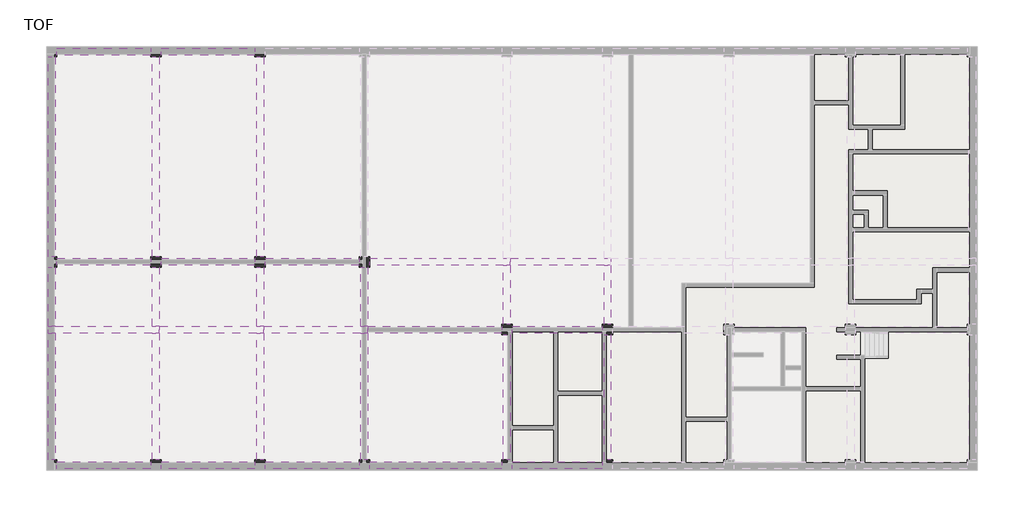
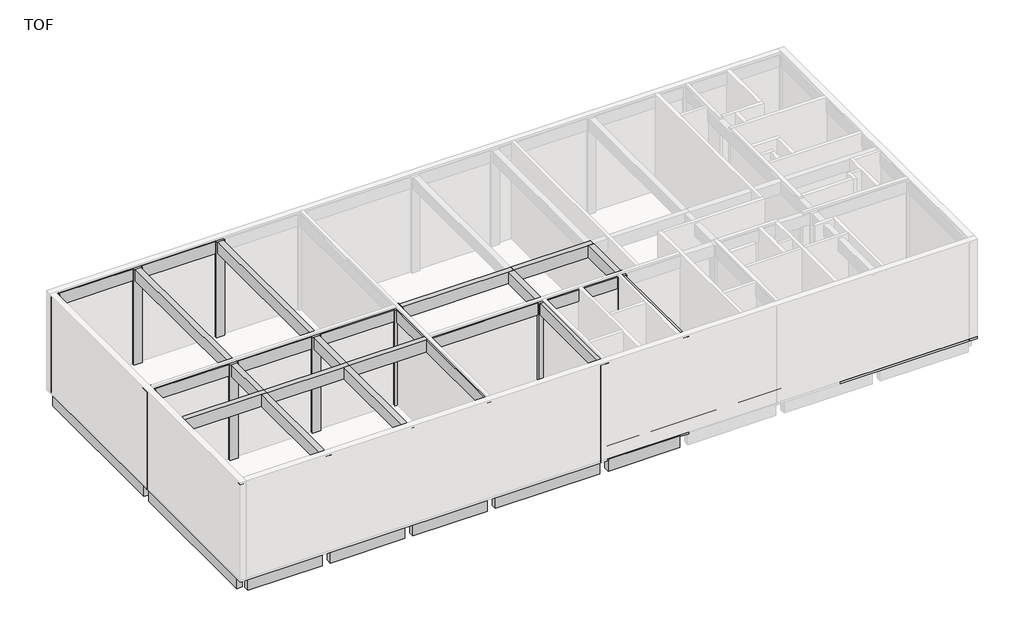
# One storey, part 2 of 3: 41 beams, 15 columns, 3 slabs.
"""IFC4 building model written with IfcOpenShell, lengths in millimetres."""

from ifc_helpers import new_model, si_unit, frame, origin, origin_with_axes, place, context, project, spatial, polyline, outline, extrude, faceted_brep, element, save

model = new_model("IFC4")

# Units and contexts
model_context = context("Model", 3, world=origin())
ifc_project = project(units=[si_unit("LENGTHUNIT", "METRE", prefix="MILLI")], contexts=[model_context])

# Site, building, storey
site = spatial("IfcSite", under=ifc_project)
building = spatial("IfcBuilding", under=site)
storey = spatial("IfcBuildingStorey", under=building, Name="TOF", Elevation=150.0)

# Beams
placement = place(None, origin())
element("IfcBeam", 1, ObjectType="RC Beam_Rectangular : H_SB_ACB_B400xH900", at=placement, inside=storey, context=model_context, shape_type="SweptSolid", body=[
    extrude(outline(polyline([(124.7, 12616.5208589), (-275.3, 12616.5208589), (-275.3, 24116.5208589), (124.7, 24116.5208589), (124.7, 12616.5208589)])), frame((0.0, 0.0, -900.0), z_axis=(0.0, 0.0, 1.0), x_axis=(1.0, 0.0, 0.0)), (0.0, 0.0, 1.0), 900.0),
])
element("IfcBeam", 2, ObjectType="RC Beam_Rectangular : H_SB_ACB_B400xH900", at=placement, inside=storey, context=model_context, shape_type="SweptSolid", body=[
    extrude(outline(polyline([(124.7, 916.5208589), (-275.3, 916.5208589), (-275.3, 12016.5208589), (124.7, 12016.5208589), (124.7, 916.5208589)])), frame((0.0, 0.0, -900.0), z_axis=(0.0, 0.0, 1.0), x_axis=(1.0, 0.0, 0.0)), (0.0, 0.0, 1.0), 900.0),
])
element("IfcBeam", 3, ObjectType="RC Beam_Rectangular : H_SB_ACB_B400xH900", at=placement, inside=storey, context=model_context, shape_type="SweptSolid", body=[
    extrude(outline(polyline([(5624.7, 24616.5208589), (5624.7, 24216.5208589), (224.7, 24216.5208589), (224.7, 24616.5208589), (5624.7, 24616.5208589)])), frame((0.0, 0.0, -900.0), z_axis=(0.0, 0.0, 1.0), x_axis=(1.0, 0.0, 0.0)), (0.0, 0.0, 1.0), 900.0),
])
element("IfcBeam", 4, ObjectType="RC Beam_Rectangular : H_SB_ACB_B400xH900", at=placement, inside=storey, context=model_context, shape_type="SweptSolid", body=[
    extrude(outline(polyline([(6224.7, 24216.5208589), (6224.7, 24616.5208589), (11624.7, 24616.5208589), (11624.7, 24216.5208589), (6224.7, 24216.5208589)])), frame((0.0, 0.0, -900.0), z_axis=(0.0, 0.0, 1.0), x_axis=(1.0, 0.0, 0.0)), (0.0, 0.0, 1.0), 900.0),
])
element("IfcBeam", 5, ObjectType="RC Beam_Rectangular : H_SB_ACB_B400xH900", at=placement, inside=storey, context=model_context, shape_type="SweptSolid", body=[
    extrude(outline(polyline([(224.7, 416.5208589), (224.7, 816.5208589), (5624.7, 816.5208589), (5624.7, 416.5208589), (224.7, 416.5208589)])), frame((0.0, 0.0, -900.0), z_axis=(0.0, 0.0, 1.0), x_axis=(1.0, 0.0, 0.0)), (0.0, 0.0, 1.0), 900.0),
])
element("IfcBeam", 6, ObjectType="RC Beam_Rectangular : H_SB_ACB_B400xH900", at=placement, inside=storey, context=model_context, shape_type="SweptSolid", body=[
    extrude(outline(polyline([(6224.7, 416.5208589), (6224.7, 816.5208589), (11624.7, 816.5208589), (11624.7, 416.5208589), (6224.7, 416.5208589)])), frame((0.0, 0.0, -900.0), z_axis=(0.0, 0.0, 1.0), x_axis=(1.0, 0.0, 0.0)), (0.0, 0.0, 1.0), 900.0),
])
element("IfcBeam", 7, ObjectType="RC Beam_Rectangular : H_SB_ACB_B400xH900", at=placement, inside=storey, context=model_context, shape_type="SweptSolid", body=[
    extrude(outline(polyline([(12224.7, 416.5208589), (12224.7, 816.5208589), (17624.7, 816.5208589), (17624.7, 416.5208589), (12224.7, 416.5208589)])), frame((0.0, 0.0, -900.0), z_axis=(0.0, 0.0, 1.0), x_axis=(1.0, 0.0, 0.0)), (0.0, 0.0, 1.0), 900.0),
])
element("IfcBeam", 8, ObjectType="RC Beam_Rectangular : H_SB_ACB_B400xH900", at=placement, inside=storey, context=model_context, shape_type="SweptSolid", body=[
    extrude(outline(polyline([(18224.7, 416.5208589), (18224.7, 816.5208589), (25824.7, 816.5208589), (25824.7, 416.5208589), (18224.7, 416.5208589)])), frame((0.0, 0.0, -900.0), z_axis=(0.0, 0.0, 1.0), x_axis=(1.0, 0.0, 0.0)), (0.0, 0.0, 1.0), 900.0),
])
element("IfcBeam", 9, ObjectType="RC Beam_Rectangular : H_SB_ACB_B400xH900", at=placement, inside=storey, context=model_context, shape_type="SweptSolid", body=[
    extrude(outline(polyline([(26424.7, 416.5208589), (26424.7, 816.5208589), (31624.7, 816.5208589), (31624.7, 416.5208589), (26424.7, 416.5208589)])), frame((0.0, 0.0, -900.0), z_axis=(0.0, 0.0, 1.0), x_axis=(1.0, 0.0, 0.0)), (0.0, 0.0, 1.0), 900.0),
])
element("IfcBeam", 10, ObjectType="RC Beam_Rectangular : H_SB_ACB_B400xH900", at=placement, inside=storey, context=model_context, shape_type="SweptSolid", body=[
    extrude(outline(polyline([(224.7, 12116.5208589), (224.7, 12516.5208589), (5624.7, 12516.5208589), (5624.7, 12116.5208589), (224.7, 12116.5208589)])), frame((0.0, 0.0, 6600.0), z_axis=(0.0, 0.0, 1.0), x_axis=(1.0, 0.0, 0.0)), (0.0, 0.0, 1.0), 900.0),
])
element("IfcBeam", 11, ObjectType="RC Beam_Rectangular : H_SB_ACB_B400xH900", at=placement, inside=storey, context=model_context, shape_type="SweptSolid", body=[
    extrude(outline(polyline([(6224.7, 12116.5208589), (6224.7, 12516.5208589), (11624.7, 12516.5208589), (11624.7, 12116.5208589), (6224.7, 12116.5208589)])), frame((0.0, 0.0, 6600.0), z_axis=(0.0, 0.0, 1.0), x_axis=(1.0, 0.0, 0.0)), (0.0, 0.0, 1.0), 900.0),
])
element("IfcBeam", 12, ObjectType="RC Beam_Rectangular : H_SB_ACB_B400xH900", at=placement, inside=storey, context=model_context, shape_type="SweptSolid", body=[
    extrude(outline(polyline([(12224.7, 12116.5208589), (12224.7, 12516.5208589), (17624.7, 12516.5208589), (17624.7, 12116.5208589), (12224.7, 12116.5208589)])), frame((0.0, 0.0, 6600.0), z_axis=(0.0, 0.0, 1.0), x_axis=(1.0, 0.0, 0.0)), (0.0, 0.0, 1.0), 900.0),
])
element("IfcBeam", 13, ObjectType="RC Beam_Rectangular : H_SB_ACB_B400xH900", at=placement, inside=storey, context=model_context, shape_type="Brep", body=[
    faceted_brep([(26324.7, 12116.5208589, 7500.0), (26324.7, 12516.5208589, 7500.0), (25924.7, 12516.5208589, 7500.0), (18224.7, 12516.5208589, 7500.0), (18224.7, 12116.5208589, 7500.0), (25924.7, 12116.5208589, 7500.0), (26324.7, 12116.5208589, 6600.0), (18224.7, 12116.5208589, 6600.0), (25924.7, 12116.5208589, 6600.0), (26324.7, 12516.5208589, 6600.0), (18224.7, 12516.5208589, 6600.0), (25924.7, 12516.5208589, 6600.0)], [[[0, 1, 2, 3, 4, 5]], [[6, 0, 5, 4, 7, 8]], [[9, 6, 8, 7, 10, 11]], [[1, 9, 11, 10, 3, 2]], [[4, 3, 10, 7]], [[1, 0, 6, 9]]]),
])
element("IfcBeam", 14, ObjectType="RC Beam_Rectangular : H_SB_ACB_B400xH900", at=placement, inside=storey, context=model_context, shape_type="Brep", body=[
    faceted_brep([(32124.7, 12116.5208589, 7500.0), (32124.7, 12516.5208589, 7500.0), (31724.7, 12516.5208589, 7500.0), (26324.7, 12516.5208589, 7500.0), (26324.7, 12116.5208589, 7500.0), (31724.7, 12116.5208589, 7500.0), (32124.7, 12116.5208589, 6600.0), (26324.7, 12116.5208589, 6600.0), (31724.7, 12116.5208589, 6600.0), (32124.7, 12516.5208589, 6600.0), (26324.7, 12516.5208589, 6600.0), (31724.7, 12516.5208589, 6600.0)], [[[0, 1, 2, 3, 4, 5]], [[6, 0, 5, 4, 7, 8]], [[9, 6, 8, 7, 10, 11]], [[1, 9, 11, 10, 3, 2]], [[1, 0, 6, 9]], [[4, 3, 10, 7]]]),
])
element("IfcBeam", 15, ObjectType="RC Beam_Rectangular : H_SB_ACB_B400xH900", at=placement, inside=storey, context=model_context, shape_type="SweptSolid", body=[
    extrude(outline(polyline([(224.7, 24216.5208589), (224.7, 24616.5208589), (5624.7, 24616.5208589), (5624.7, 24216.5208589), (224.7, 24216.5208589)])), frame((0.0, 0.0, 6600.0), z_axis=(0.0, 0.0, 1.0), x_axis=(1.0, 0.0, 0.0)), (0.0, 0.0, 1.0), 900.0),
])
element("IfcBeam", 16, ObjectType="RC Beam_Rectangular : H_SB_ACB_B400xH900", at=placement, inside=storey, context=model_context, shape_type="SweptSolid", body=[
    extrude(outline(polyline([(6224.7, 24216.5208589), (6224.7, 24616.5208589), (11624.7, 24616.5208589), (11624.7, 24216.5208589), (6224.7, 24216.5208589)])), frame((0.0, 0.0, 6600.0), z_axis=(0.0, 0.0, 1.0), x_axis=(1.0, 0.0, 0.0)), (0.0, 0.0, 1.0), 900.0),
])
element("IfcBeam", 17, ObjectType="RC Beam_Rectangular : H_SB_ACB_B400xH900", at=placement, inside=storey, context=model_context, shape_type="Brep", body=[
    faceted_brep([(-275.3, 8616.5208589, 7500.0), (-275.3, 8216.5208589, 7500.0), (124.7, 8216.5208589, 7500.0), (5724.7, 8216.5208589, 7500.0), (6124.7, 8216.5208589, 7500.0), (6124.7, 8616.5208589, 7500.0), (5724.7, 8616.5208589, 7500.0), (124.7, 8616.5208589, 7500.0), (-275.3, 8216.5208589, 6600.0), (124.7, 8216.5208589, 6600.0), (5724.7, 8216.5208589, 6600.0), (6124.7, 8216.5208589, 6600.0), (-275.3, 8616.5208589, 6600.0), (124.7, 8616.5208589, 6600.0), (5724.7, 8616.5208589, 6600.0), (6124.7, 8616.5208589, 6600.0)], [[[0, 1, 2, 3, 4, 5, 6, 7]], [[1, 8, 9, 10, 11, 4, 3, 2]], [[8, 12, 13, 14, 15, 11, 10, 9]], [[12, 0, 7, 6, 5, 15, 14, 13]], [[1, 0, 12, 8]], [[5, 4, 11, 15]]]),
])
element("IfcBeam", 18, ObjectType="RC Beam_Rectangular : H_SB_ACB_B400xH900", at=placement, inside=storey, context=model_context, shape_type="Brep", body=[
    faceted_brep([(12124.7, 8216.5208589, 7500.0), (12124.7, 8616.5208589, 7500.0), (11724.7, 8616.5208589, 7500.0), (6124.7, 8616.5208589, 7500.0), (6124.7, 8216.5208589, 7500.0), (11724.7, 8216.5208589, 7500.0), (12124.7, 8216.5208589, 6600.0), (6124.7, 8216.5208589, 6600.0), (11724.7, 8216.5208589, 6600.0), (12124.7, 8616.5208589, 6600.0), (6124.7, 8616.5208589, 6600.0), (11724.7, 8616.5208589, 6600.0)], [[[0, 1, 2, 3, 4, 5]], [[6, 0, 5, 4, 7, 8]], [[9, 6, 8, 7, 10, 11]], [[1, 9, 11, 10, 3, 2]], [[1, 0, 6, 9]], [[4, 3, 10, 7]]]),
])
element("IfcBeam", 19, ObjectType="RC Beam_Rectangular : H_SB_ACB_B400xH900", at=placement, inside=storey, context=model_context, shape_type="Brep", body=[
    faceted_brep([(18124.7, 8216.5208589, 7500.0), (18124.7, 8616.5208589, 7500.0), (17724.7, 8616.5208589, 7500.0), (12124.7, 8616.5208589, 7500.0), (12124.7, 8216.5208589, 7500.0), (17724.7, 8216.5208589, 7500.0), (18124.7, 8216.5208589, 6600.0), (12124.7, 8216.5208589, 6600.0), (17724.7, 8216.5208589, 6600.0), (18124.7, 8616.5208589, 6600.0), (12124.7, 8616.5208589, 6600.0), (17724.7, 8616.5208589, 6600.0)], [[[0, 1, 2, 3, 4, 5]], [[6, 0, 5, 4, 7, 8]], [[9, 6, 8, 7, 10, 11]], [[1, 9, 11, 10, 3, 2]], [[1, 0, 6, 9]], [[4, 3, 10, 7]]]),
])
element("IfcBeam", 20, ObjectType="RC Beam_Rectangular : H_SB_ACB_B400xH900", at=placement, inside=storey, context=model_context, shape_type="SweptSolid", body=[
    extrude(outline(polyline([(18124.7, 8216.5208589), (18124.7, 8616.5208589), (25824.7, 8616.5208589), (25824.7, 8216.5208589), (18124.7, 8216.5208589)])), frame((0.0, 0.0, 6600.0), z_axis=(0.0, 0.0, 1.0), x_axis=(1.0, 0.0, 0.0)), (0.0, 0.0, 1.0), 900.0),
])
element("IfcBeam", 21, ObjectType="RC Beam_Rectangular : H_SB_ACB_B400xH900", at=placement, inside=storey, context=model_context, shape_type="SweptSolid", body=[
    extrude(outline(polyline([(26424.7, 8216.5208589), (26424.7, 8616.5208589), (31624.7, 8616.5208589), (31624.7, 8216.5208589), (26424.7, 8216.5208589)])), frame((0.0, 0.0, 6600.0), z_axis=(0.0, 0.0, 1.0), x_axis=(1.0, 0.0, 0.0)), (0.0, 0.0, 1.0), 900.0),
])
element("IfcBeam", 22, ObjectType="RC Beam_Rectangular : H_SB_ACB_B400xH900", at=placement, inside=storey, context=model_context, shape_type="SweptSolid", body=[
    extrude(outline(polyline([(224.7, 416.5208589), (224.7, 816.5208589), (5624.7, 816.5208589), (5624.7, 416.5208589), (224.7, 416.5208589)])), frame((0.0, 0.0, 6600.0), z_axis=(0.0, 0.0, 1.0), x_axis=(1.0, 0.0, 0.0)), (0.0, 0.0, 1.0), 900.0),
])
element("IfcBeam", 23, ObjectType="RC Beam_Rectangular : H_SB_ACB_B400xH900", at=placement, inside=storey, context=model_context, shape_type="SweptSolid", body=[
    extrude(outline(polyline([(6224.7, 416.5208589), (6224.7, 816.5208589), (11624.7, 816.5208589), (11624.7, 416.5208589), (6224.7, 416.5208589)])), frame((0.0, 0.0, 6600.0), z_axis=(0.0, 0.0, 1.0), x_axis=(1.0, 0.0, 0.0)), (0.0, 0.0, 1.0), 900.0),
])
element("IfcBeam", 24, ObjectType="RC Beam_Rectangular : H_SB_ACB_B400xH900", at=placement, inside=storey, context=model_context, shape_type="SweptSolid", body=[
    extrude(outline(polyline([(12224.7, 416.5208589), (12224.7, 816.5208589), (17624.7, 816.5208589), (17624.7, 416.5208589), (12224.7, 416.5208589)])), frame((0.0, 0.0, 6600.0), z_axis=(0.0, 0.0, 1.0), x_axis=(1.0, 0.0, 0.0)), (0.0, 0.0, 1.0), 900.0),
])
element("IfcBeam", 25, ObjectType="RC Beam_Rectangular : H_SB_ACB_B400xH900", at=placement, inside=storey, context=model_context, shape_type="SweptSolid", body=[
    extrude(outline(polyline([(18224.7, 416.5208589), (18224.7, 816.5208589), (25824.7, 816.5208589), (25824.7, 416.5208589), (18224.7, 416.5208589)])), frame((0.0, 0.0, 6600.0), z_axis=(0.0, 0.0, 1.0), x_axis=(1.0, 0.0, 0.0)), (0.0, 0.0, 1.0), 900.0),
])
element("IfcBeam", 26, ObjectType="RC Beam_Rectangular : H_SB_ACB_B400xH900", at=placement, inside=storey, context=model_context, shape_type="SweptSolid", body=[
    extrude(outline(polyline([(26424.7, 416.5208589), (26424.7, 816.5208589), (31624.7, 816.5208589), (31624.7, 416.5208589), (26424.7, 416.5208589)])), frame((0.0, 0.0, 6600.0), z_axis=(0.0, 0.0, 1.0), x_axis=(1.0, 0.0, 0.0)), (0.0, 0.0, 1.0), 900.0),
])
element("IfcBeam", 27, ObjectType="RC Beam_Rectangular : H_SB_ACB_B400xH900", at=placement, inside=storey, context=model_context, shape_type="SweptSolid", body=[
    extrude(outline(polyline([(-275.3, 8216.5208589), (124.7, 8216.5208589), (124.7, 916.5208589), (-275.3, 916.5208589), (-275.3, 8216.5208589)])), frame((0.0, 0.0, 6600.0), z_axis=(0.0, 0.0, 1.0), x_axis=(1.0, 0.0, 0.0)), (0.0, 0.0, 1.0), 900.0),
])
element("IfcBeam", 28, ObjectType="RC Beam_Rectangular : H_SB_ACB_B400xH900", at=placement, inside=storey, context=model_context, shape_type="SweptSolid", body=[
    extrude(outline(polyline([(124.7, 8616.5208589), (-275.3, 8616.5208589), (-275.3, 12016.5208589), (124.7, 12016.5208589), (124.7, 8616.5208589)])), frame((0.0, 0.0, 6600.0), z_axis=(0.0, 0.0, 1.0), x_axis=(1.0, 0.0, 0.0)), (0.0, 0.0, 1.0), 900.0),
])
element("IfcBeam", 29, ObjectType="RC Beam_Rectangular : H_SB_ACB_B400xH900", at=placement, inside=storey, context=model_context, shape_type="SweptSolid", body=[
    extrude(outline(polyline([(124.7, 12616.5208589), (-275.3, 12616.5208589), (-275.3, 24116.5208589), (124.7, 24116.5208589), (124.7, 12616.5208589)])), frame((0.0, 0.0, 6600.0), z_axis=(0.0, 0.0, 1.0), x_axis=(1.0, 0.0, 0.0)), (0.0, 0.0, 1.0), 900.0),
])
element("IfcBeam", 30, ObjectType="RC Beam_Rectangular : H_SB_ACB_B400xH900", at=placement, inside=storey, context=model_context, shape_type="SweptSolid", body=[
    extrude(outline(polyline([(5724.7, 8216.5208589), (6124.7, 8216.5208589), (6124.7, 916.5208589), (5724.7, 916.5208589), (5724.7, 8216.5208589)])), frame((0.0, 0.0, 6600.0), z_axis=(0.0, 0.0, 1.0), x_axis=(1.0, 0.0, 0.0)), (0.0, 0.0, 1.0), 900.0),
])
element("IfcBeam", 31, ObjectType="RC Beam_Rectangular : H_SB_ACB_B400xH900", at=placement, inside=storey, context=model_context, shape_type="SweptSolid", body=[
    extrude(outline(polyline([(6124.7, 8616.5208589), (5724.7, 8616.5208589), (5724.7, 12016.5208589), (6124.7, 12016.5208589), (6124.7, 8616.5208589)])), frame((0.0, 0.0, 6600.0), z_axis=(0.0, 0.0, 1.0), x_axis=(1.0, 0.0, 0.0)), (0.0, 0.0, 1.0), 900.0),
])
element("IfcBeam", 32, ObjectType="RC Beam_Rectangular : H_SB_ACB_B400xH900", at=placement, inside=storey, context=model_context, shape_type="SweptSolid", body=[
    extrude(outline(polyline([(6124.7, 12616.5208589), (5724.7, 12616.5208589), (5724.7, 24116.5208589), (6124.7, 24116.5208589), (6124.7, 12616.5208589)])), frame((0.0, 0.0, 6600.0), z_axis=(0.0, 0.0, 1.0), x_axis=(1.0, 0.0, 0.0)), (0.0, 0.0, 1.0), 900.0),
])
element("IfcBeam", 33, ObjectType="RC Beam_Rectangular : H_SB_ACB_B400xH900", at=placement, inside=storey, context=model_context, shape_type="SweptSolid", body=[
    extrude(outline(polyline([(11724.7, 8216.5208589), (12124.7, 8216.5208589), (12124.7, 916.5208589), (11724.7, 916.5208589), (11724.7, 8216.5208589)])), frame((0.0, 0.0, 6600.0), z_axis=(0.0, 0.0, 1.0), x_axis=(1.0, 0.0, 0.0)), (0.0, 0.0, 1.0), 900.0),
])
element("IfcBeam", 34, ObjectType="RC Beam_Rectangular : H_SB_ACB_B400xH900", at=placement, inside=storey, context=model_context, shape_type="SweptSolid", body=[
    extrude(outline(polyline([(12124.7, 8616.5208589), (11724.7, 8616.5208589), (11724.7, 12016.5208589), (12124.7, 12016.5208589), (12124.7, 8616.5208589)])), frame((0.0, 0.0, 6600.0), z_axis=(0.0, 0.0, 1.0), x_axis=(1.0, 0.0, 0.0)), (0.0, 0.0, 1.0), 900.0),
])
element("IfcBeam", 35, ObjectType="RC Beam_Rectangular : H_SB_ACB_B400xH900", at=placement, inside=storey, context=model_context, shape_type="SweptSolid", body=[
    extrude(outline(polyline([(12124.7, 12616.5208589), (11724.7, 12616.5208589), (11724.7, 24116.5208589), (12124.7, 24116.5208589), (12124.7, 12616.5208589)])), frame((0.0, 0.0, 6600.0), z_axis=(0.0, 0.0, 1.0), x_axis=(1.0, 0.0, 0.0)), (0.0, 0.0, 1.0), 900.0),
])
element("IfcBeam", 36, ObjectType="RC Beam_Rectangular : H_SB_ACB_B400xH900", at=placement, inside=storey, context=model_context, shape_type="SweptSolid", body=[
    extrude(outline(polyline([(17724.7, 8216.5208589), (18124.7, 8216.5208589), (18124.7, 916.5208589), (17724.7, 916.5208589), (17724.7, 8216.5208589)])), frame((0.0, 0.0, 6600.0), z_axis=(0.0, 0.0, 1.0), x_axis=(1.0, 0.0, 0.0)), (0.0, 0.0, 1.0), 900.0),
])
element("IfcBeam", 37, ObjectType="RC Beam_Rectangular : H_SB_ACB_B400xH900", at=placement, inside=storey, context=model_context, shape_type="SweptSolid", body=[
    extrude(outline(polyline([(18124.7, 8616.5208589), (17724.7, 8616.5208589), (17724.7, 12016.5208589), (18124.7, 12016.5208589), (18124.7, 8616.5208589)])), frame((0.0, 0.0, 6600.0), z_axis=(0.0, 0.0, 1.0), x_axis=(1.0, 0.0, 0.0)), (0.0, 0.0, 1.0), 900.0),
])
element("IfcBeam", 38, ObjectType="RC Beam_Rectangular : H_SB_ACB_B400xH900", at=placement, inside=storey, context=model_context, shape_type="SweptSolid", body=[
    extrude(outline(polyline([(25924.7, 8116.5208589), (26324.7, 8116.5208589), (26324.7, 916.5208589), (25924.7, 916.5208589), (25924.7, 8116.5208589)])), frame((0.0, 0.0, 6600.0), z_axis=(0.0, 0.0, 1.0), x_axis=(1.0, 0.0, 0.0)), (0.0, 0.0, 1.0), 900.0),
])
element("IfcBeam", 39, ObjectType="RC Beam_Rectangular : H_SB_ACB_B400xH900", at=placement, inside=storey, context=model_context, shape_type="SweptSolid", body=[
    extrude(outline(polyline([(25924.7, 12116.5208589), (26324.7, 12116.5208589), (26324.7, 8716.5208589), (25924.7, 8716.5208589), (25924.7, 12116.5208589)])), frame((0.0, 0.0, 6600.0), z_axis=(0.0, 0.0, 1.0), x_axis=(1.0, 0.0, 0.0)), (0.0, 0.0, 1.0), 900.0),
])
element("IfcBeam", 40, ObjectType="RC Beam_Rectangular : H_SB_ACB_B400xH900", at=placement, inside=storey, context=model_context, shape_type="SweptSolid", body=[
    extrude(outline(polyline([(31724.7, 8116.5208589), (32124.7, 8116.5208589), (32124.7, 916.5208589), (31724.7, 916.5208589), (31724.7, 8116.5208589)])), frame((0.0, 0.0, 6600.0), z_axis=(0.0, 0.0, 1.0), x_axis=(1.0, 0.0, 0.0)), (0.0, 0.0, 1.0), 900.0),
])
element("IfcBeam", 41, ObjectType="RC Beam_Rectangular : H_SB_ACB_B400xH900", at=placement, inside=storey, context=model_context, shape_type="SweptSolid", body=[
    extrude(outline(polyline([(31724.7, 12116.5208589), (32124.7, 12116.5208589), (32124.7, 8716.5208589), (31724.7, 8716.5208589), (31724.7, 12116.5208589)])), frame((0.0, 0.0, 6600.0), z_axis=(0.0, 0.0, 1.0), x_axis=(1.0, 0.0, 0.0)), (0.0, 0.0, 1.0), 900.0),
])

# Columns
element("IfcColumn", 42, ObjectType="RC_Column_Rectangular : H_SC_ACC_W600xL600", at=placement, inside=storey, context=model_context, shape_type="Brep", body=[
    faceted_brep([(224.7, 12016.5208589, 0.0), (-375.3, 12016.5208589, 0.0), (-375.3, 12316.5208589, 0.0), (224.7, 12316.5208589, 0.0), (224.7, 12616.5208589, 7500.0), (224.7, 12516.5208589, 7500.0), (224.7, 12116.5208589, 7500.0), (224.7, 12016.5208589, 7500.0), (224.7, 12316.5208589, 150.0), (224.7, 12616.5208589, 150.0), (124.7, 12016.5208589, 7500.0), (-275.3, 12016.5208589, 7500.0), (-375.3, 12016.5208589, 7500.0), (-375.3, 12616.5208589, 7500.0), (-375.3, 12616.5208589, 150.0), (-375.3, 12316.5208589, 150.0), (-275.3, 12616.5208589, 7500.0), (124.7, 12616.5208589, 7500.0)], [[[0, 1, 2, 3]], [[4, 5, 6, 7, 0, 3, 8, 9]], [[1, 0, 7, 10, 11, 12]], [[1, 12, 13, 14, 15, 2]], [[13, 16, 17, 4, 9, 14]], [[7, 6, 5, 4, 17, 16, 13, 12, 11, 10]], [[8, 15, 14, 9]], [[15, 8, 3, 2]]]),
])
element("IfcColumn", 43, ObjectType="RC_Column_Rectangular : H_SC_ACC_W600xL600", at=placement, inside=storey, context=model_context, shape_type="Brep", body=[
    faceted_brep([(6224.7, 12016.5208589, 0.0), (5624.7, 12016.5208589, 0.0), (5624.7, 12316.5208589, 0.0), (6224.7, 12316.5208589, 0.0), (6224.7, 12616.5208589, 7500.0), (6224.7, 12516.5208589, 7500.0), (6224.7, 12116.5208589, 7500.0), (6224.7, 12016.5208589, 7500.0), (6224.7, 12316.5208589, 150.0), (6224.7, 12616.5208589, 150.0), (6124.7, 12016.5208589, 7500.0), (5724.7, 12016.5208589, 7500.0), (5624.7, 12016.5208589, 7500.0), (5624.7, 12116.5208589, 7500.0), (5624.7, 12516.5208589, 7500.0), (5624.7, 12616.5208589, 7500.0), (5624.7, 12616.5208589, 150.0), (5624.7, 12316.5208589, 150.0), (5724.7, 12616.5208589, 7500.0), (6124.7, 12616.5208589, 7500.0)], [[[0, 1, 2, 3]], [[4, 5, 6, 7, 0, 3, 8, 9]], [[1, 0, 7, 10, 11, 12]], [[1, 12, 13, 14, 15, 16, 17, 2]], [[15, 18, 19, 4, 9, 16]], [[7, 6, 5, 4, 19, 18, 15, 14, 13, 12, 11, 10]], [[8, 17, 16, 9]], [[17, 8, 3, 2]]]),
])
element("IfcColumn", 44, ObjectType="RC_Column_Rectangular : H_SC_ACC_W600xL600", at=placement, inside=storey, context=model_context, shape_type="Brep", body=[
    faceted_brep([(12224.7, 12016.5208589, 0.0), (11624.7, 12016.5208589, 0.0), (11624.7, 12316.5208589, 0.0), (12224.7, 12316.5208589, 0.0), (12224.7, 12616.5208589, 7500.0), (12224.7, 12516.5208589, 7500.0), (12224.7, 12116.5208589, 7500.0), (12224.7, 12016.5208589, 7500.0), (12224.7, 12316.5208589, 150.0), (12224.7, 12616.5208589, 150.0), (12124.7, 12016.5208589, 7500.0), (11724.7, 12016.5208589, 7500.0), (11624.7, 12016.5208589, 7500.0), (11624.7, 12116.5208589, 7500.0), (11624.7, 12516.5208589, 7500.0), (11624.7, 12616.5208589, 7500.0), (11624.7, 12616.5208589, 150.0), (11624.7, 12316.5208589, 150.0), (11724.7, 12616.5208589, 7500.0), (12124.7, 12616.5208589, 7500.0)], [[[0, 1, 2, 3]], [[4, 5, 6, 7, 0, 3, 8, 9]], [[1, 0, 7, 10, 11, 12]], [[1, 12, 13, 14, 15, 16, 17, 2]], [[15, 18, 19, 4, 9, 16]], [[7, 6, 5, 4, 19, 18, 15, 14, 13, 12, 11, 10]], [[8, 17, 16, 9]], [[17, 8, 3, 2]]]),
])
element("IfcColumn", 45, ObjectType="RC_Column_Rectangular : H_SC_ACC_W600xL600", at=placement, inside=storey, context=model_context, shape_type="Brep", body=[
    faceted_brep([(17924.7, 12016.5208589, 0.0), (17624.7, 12016.5208589, 0.0), (17624.7, 12316.5208589, 0.0), (17924.7, 12316.5208589, 0.0), (18224.7, 12616.5208589, 7500.0), (18224.7, 12516.5208589, 7500.0), (18224.7, 12116.5208589, 7500.0), (18224.7, 12016.5208589, 7500.0), (18224.7, 12016.5208589, 150.0), (18224.7, 12616.5208589, 150.0), (18124.7, 12016.5208589, 7500.0), (17724.7, 12016.5208589, 7500.0), (17624.7, 12016.5208589, 7500.0), (17924.7, 12016.5208589, 150.0), (17624.7, 12116.5208589, 7500.0), (17624.7, 12516.5208589, 7500.0), (17624.7, 12616.5208589, 7500.0), (17624.7, 12616.5208589, 150.0), (17624.7, 12316.5208589, 150.0), (17724.7, 12616.5208589, 7500.0), (18124.7, 12616.5208589, 7500.0), (17924.7, 12316.5208589, 150.0)], [[[0, 1, 2, 3]], [[4, 5, 6, 7, 8, 9]], [[7, 10, 11, 12, 1, 0, 13, 8]], [[1, 12, 14, 15, 16, 17, 18, 2]], [[16, 19, 20, 4, 9, 17]], [[7, 6, 5, 4, 20, 19, 16, 15, 14, 12, 11, 10]], [[13, 21, 18, 17, 9, 8]], [[3, 21, 13, 0]], [[21, 3, 2, 18]]]),
])
element("IfcColumn", 46, ObjectType="RC_Column_Rectangular : H_SC_ACC_W600xL600", at=placement, inside=storey, context=model_context, shape_type="Brep", body=[
    faceted_brep([(224.7, 24716.5208589, 7500.0), (224.7, 24616.5208589, 7500.0), (224.7, 24216.5208589, 7500.0), (224.7, 24116.5208589, 7500.0), (224.7, 24116.5208589, 150.0), (224.7, 24716.5208589, 150.0), (124.7, 24116.5208589, 7500.0), (-275.3, 24116.5208589, 7500.0), (-375.3, 24116.5208589, 7500.0), (-375.3, 24116.5208589, 150.0), (-375.3, 24716.5208589, 7500.0), (-375.3, 24716.5208589, 150.0)], [[[0, 1, 2, 3, 4, 5]], [[3, 6, 7, 8, 9, 4]], [[8, 10, 11, 9]], [[10, 0, 5, 11]], [[3, 2, 1, 0, 10, 8, 7, 6]], [[5, 4, 9, 11]]]),
])
element("IfcColumn", 47, ObjectType="RC_Column_Rectangular : H_SC_ACC_W600xL600", at=placement, inside=storey, context=model_context, shape_type="Brep", body=[
    faceted_brep([(6224.7, 24716.5208589, 7500.0), (6224.7, 24616.5208589, 7500.0), (6224.7, 24216.5208589, 7500.0), (6224.7, 24116.5208589, 7500.0), (6224.7, 24116.5208589, 150.0), (6224.7, 24716.5208589, 150.0), (6124.7, 24116.5208589, 7500.0), (5724.7, 24116.5208589, 7500.0), (5624.7, 24116.5208589, 7500.0), (5624.7, 24116.5208589, 150.0), (5624.7, 24216.5208589, 7500.0), (5624.7, 24616.5208589, 7500.0), (5624.7, 24716.5208589, 7500.0), (5624.7, 24716.5208589, 150.0)], [[[0, 1, 2, 3, 4, 5]], [[3, 6, 7, 8, 9, 4]], [[8, 10, 11, 12, 13, 9]], [[12, 0, 5, 13]], [[3, 2, 1, 0, 12, 11, 10, 8, 7, 6]], [[5, 4, 9, 13]]]),
])
element("IfcColumn", 48, ObjectType="RC_Column_Rectangular : H_SC_ACC_W600xL600", at=placement, inside=storey, context=model_context, shape_type="Brep", body=[
    faceted_brep([(12224.7, 24716.5208589, 7500.0), (12224.7, 24616.5208589, 7500.0), (12224.7, 24216.5208589, 7500.0), (12224.7, 24116.5208589, 7500.0), (12224.7, 24116.5208589, 150.0), (12224.7, 24716.5208589, 150.0), (12124.7, 24116.5208589, 7500.0), (11724.7, 24116.5208589, 7500.0), (11624.7, 24116.5208589, 7500.0), (11624.7, 24116.5208589, 150.0), (11624.7, 24216.5208589, 7500.0), (11624.7, 24616.5208589, 7500.0), (11624.7, 24716.5208589, 7500.0), (11624.7, 24716.5208589, 150.0)], [[[0, 1, 2, 3, 4, 5]], [[3, 6, 7, 8, 9, 4]], [[8, 10, 11, 12, 13, 9]], [[12, 0, 5, 13]], [[3, 2, 1, 0, 12, 11, 10, 8, 7, 6]], [[5, 4, 9, 13]]]),
])
element("IfcColumn", 49, ObjectType="RC_Column_Rectangular : H_SC_ACC_W600xL600", at=placement, inside=storey, context=model_context, shape_type="Brep", body=[
    faceted_brep([(26424.7, 8116.5208589, 0.0), (25824.7, 8116.5208589, 0.0), (25824.7, 8416.5208589, 0.0), (26424.7, 8416.5208589, 0.0), (26424.7, 8716.5208589, 7500.0), (26424.7, 8616.5208589, 7500.0), (26424.7, 8216.5208589, 7500.0), (26424.7, 8116.5208589, 7500.0), (26424.7, 8416.5208589, 150.0), (26424.7, 8716.5208589, 150.0), (26324.7, 8116.5208589, 7500.0), (25924.7, 8116.5208589, 7500.0), (25824.7, 8116.5208589, 7500.0), (25824.7, 8216.5208589, 7500.0), (25824.7, 8616.5208589, 7500.0), (25824.7, 8716.5208589, 7500.0), (25824.7, 8716.5208589, 150.0), (25824.7, 8416.5208589, 150.0), (25924.7, 8716.5208589, 7500.0), (26324.7, 8716.5208589, 7500.0)], [[[0, 1, 2, 3]], [[4, 5, 6, 7, 0, 3, 8, 9]], [[1, 0, 7, 10, 11, 12]], [[1, 12, 13, 14, 15, 16, 17, 2]], [[15, 18, 19, 4, 9, 16]], [[7, 6, 5, 4, 19, 18, 15, 14, 13, 12, 11, 10]], [[8, 17, 16, 9]], [[17, 8, 3, 2]]]),
])
element("IfcColumn", 50, ObjectType="RC_Column_Rectangular : H_SC_ACC_W600xL600", at=placement, inside=storey, context=model_context, shape_type="Brep", body=[
    faceted_brep([(32224.7, 8116.5208589, 0.0), (31624.7, 8116.5208589, 0.0), (31624.7, 8416.5208589, 0.0), (32224.7, 8416.5208589, 0.0), (32224.7, 8716.5208589, 7500.0), (32224.7, 8616.5208589, 7500.0), (32224.7, 8216.5208589, 7500.0), (32224.7, 8116.5208589, 7500.0), (32224.7, 8416.5208589, 150.0), (32224.7, 8716.5208589, 150.0), (32124.7, 8116.5208589, 7500.0), (31724.7, 8116.5208589, 7500.0), (31624.7, 8116.5208589, 7500.0), (31624.7, 8216.5208589, 7500.0), (31624.7, 8616.5208589, 7500.0), (31624.7, 8716.5208589, 7500.0), (31624.7, 8716.5208589, 150.0), (31624.7, 8416.5208589, 150.0), (31724.7, 8716.5208589, 7500.0), (32124.7, 8716.5208589, 7500.0)], [[[0, 1, 2, 3]], [[4, 5, 6, 7, 0, 3, 8, 9]], [[1, 0, 7, 10, 11, 12]], [[1, 12, 13, 14, 15, 16, 17, 2]], [[15, 18, 19, 4, 9, 16]], [[7, 6, 5, 4, 19, 18, 15, 14, 13, 12, 11, 10]], [[8, 17, 16, 9]], [[17, 8, 3, 2]]]),
])
element("IfcColumn", 51, ObjectType="RC_Column_Rectangular : H_SC_ACC_W600xL600", at=placement, inside=storey, context=model_context, shape_type="Brep", body=[
    faceted_brep([(224.7, 916.5208589, 0.0), (224.7, 316.5208589, 0.0), (-375.3, 316.5208589, 0.0), (-375.3, 916.5208589, 0.0), (224.7, 916.5208589, 7500.0), (224.7, 816.5208589, 7500.0), (224.7, 416.5208589, 7500.0), (224.7, 316.5208589, 7500.0), (-375.3, 316.5208589, 7500.0), (-375.3, 916.5208589, 7500.0), (-275.3, 916.5208589, 7500.0), (124.7, 916.5208589, 7500.0)], [[[0, 1, 2, 3]], [[4, 5, 6, 7, 1, 0]], [[7, 8, 2, 1]], [[8, 9, 3, 2]], [[9, 10, 11, 4, 0, 3]], [[4, 11, 10, 9, 8, 7, 6, 5]]]),
])
element("IfcColumn", 52, ObjectType="RC_Column_Rectangular : H_SC_ACC_W600xL600", at=placement, inside=storey, context=model_context, shape_type="Brep", body=[
    faceted_brep([(6224.7, 916.5208589, 0.0), (6224.7, 316.5208589, 0.0), (5624.7, 316.5208589, 0.0), (5624.7, 916.5208589, 0.0), (6224.7, 916.5208589, 7500.0), (6224.7, 816.5208589, 7500.0), (6224.7, 416.5208589, 7500.0), (6224.7, 316.5208589, 7500.0), (5624.7, 316.5208589, 7500.0), (5624.7, 416.5208589, 7500.0), (5624.7, 816.5208589, 7500.0), (5624.7, 916.5208589, 7500.0), (5724.7, 916.5208589, 7500.0), (6124.7, 916.5208589, 7500.0)], [[[0, 1, 2, 3]], [[4, 5, 6, 7, 1, 0]], [[7, 8, 2, 1]], [[8, 9, 10, 11, 3, 2]], [[11, 12, 13, 4, 0, 3]], [[4, 13, 12, 11, 10, 9, 8, 7, 6, 5]]]),
])
element("IfcColumn", 53, ObjectType="RC_Column_Rectangular : H_SC_ACC_W600xL600", at=placement, inside=storey, context=model_context, shape_type="Brep", body=[
    faceted_brep([(12224.7, 916.5208589, 0.0), (12224.7, 316.5208589, 0.0), (11624.7, 316.5208589, 0.0), (11624.7, 916.5208589, 0.0), (12224.7, 916.5208589, 7500.0), (12224.7, 816.5208589, 7500.0), (12224.7, 416.5208589, 7500.0), (12224.7, 316.5208589, 7500.0), (11624.7, 316.5208589, 7500.0), (11624.7, 416.5208589, 7500.0), (11624.7, 816.5208589, 7500.0), (11624.7, 916.5208589, 7500.0), (11724.7, 916.5208589, 7500.0), (12124.7, 916.5208589, 7500.0)], [[[0, 1, 2, 3]], [[4, 5, 6, 7, 1, 0]], [[7, 8, 2, 1]], [[8, 9, 10, 11, 3, 2]], [[11, 12, 13, 4, 0, 3]], [[4, 13, 12, 11, 10, 9, 8, 7, 6, 5]]]),
])
element("IfcColumn", 54, ObjectType="RC_Column_Rectangular : H_SC_ACC_W600xL600", at=placement, inside=storey, context=model_context, shape_type="Brep", body=[
    faceted_brep([(18224.7, 916.5208589, 0.0), (18224.7, 316.5208589, 0.0), (17624.7, 316.5208589, 0.0), (17624.7, 916.5208589, 0.0), (18224.7, 916.5208589, 7500.0), (18224.7, 816.5208589, 7500.0), (18224.7, 416.5208589, 7500.0), (18224.7, 316.5208589, 7500.0), (17624.7, 316.5208589, 7500.0), (17624.7, 416.5208589, 7500.0), (17624.7, 816.5208589, 7500.0), (17624.7, 916.5208589, 7500.0), (17724.7, 916.5208589, 7500.0), (18124.7, 916.5208589, 7500.0)], [[[0, 1, 2, 3]], [[4, 5, 6, 7, 1, 0]], [[7, 8, 2, 1]], [[8, 9, 10, 11, 3, 2]], [[11, 12, 13, 4, 0, 3]], [[4, 13, 12, 11, 10, 9, 8, 7, 6, 5]]]),
])
element("IfcColumn", 55, ObjectType="RC_Column_Rectangular : H_SC_ACC_W600xL600", at=placement, inside=storey, context=model_context, shape_type="Brep", body=[
    faceted_brep([(26424.7, 916.5208589, 0.0), (26424.7, 316.5208589, 0.0), (25824.7, 316.5208589, 0.0), (25824.7, 916.5208589, 0.0), (26424.7, 916.5208589, 7500.0), (26424.7, 816.5208589, 7500.0), (26424.7, 416.5208589, 7500.0), (26424.7, 316.5208589, 7500.0), (25824.7, 316.5208589, 7500.0), (25824.7, 416.5208589, 7500.0), (25824.7, 816.5208589, 7500.0), (25824.7, 916.5208589, 7500.0), (25924.7, 916.5208589, 7500.0), (26324.7, 916.5208589, 7500.0)], [[[0, 1, 2, 3]], [[4, 5, 6, 7, 1, 0]], [[7, 8, 2, 1]], [[8, 9, 10, 11, 3, 2]], [[11, 12, 13, 4, 0, 3]], [[4, 13, 12, 11, 10, 9, 8, 7, 6, 5]]]),
])
element("IfcColumn", 56, ObjectType="RC_Column_Rectangular : H_SC_ACC_W600xL600", at=placement, inside=storey, context=model_context, shape_type="Brep", body=[
    faceted_brep([(32224.7, 916.5208589, 0.0), (32224.7, 316.5208589, 0.0), (31624.7, 316.5208589, 0.0), (31624.7, 916.5208589, 0.0), (32224.7, 916.5208589, 7500.0), (32224.7, 816.5208589, 7500.0), (32224.7, 416.5208589, 7500.0), (32224.7, 316.5208589, 7500.0), (31624.7, 316.5208589, 7500.0), (31624.7, 416.5208589, 7500.0), (31624.7, 816.5208589, 7500.0), (31624.7, 916.5208589, 7500.0), (31724.7, 916.5208589, 7500.0), (32124.7, 916.5208589, 7500.0)], [[[0, 1, 2, 3]], [[4, 5, 6, 7, 1, 0]], [[7, 8, 2, 1]], [[8, 9, 10, 11, 3, 2]], [[11, 12, 13, 4, 0, 3]], [[4, 13, 12, 11, 10, 9, 8, 7, 6, 5]]]),
])

# Slabs
element("IfcSlab", 57, ObjectType="H_FL_AMF_RC Slab_T150", at=placement, inside=storey, context=model_context, shape_type="Brep", body=[
    faceted_brep([(53224.7, 11850.5208589, 1000.0), (50777.7, 11850.5208589, 1000.0), (50777.7, 8416.5208589, 1000.0), (46624.7, 8416.5208589, 1000.0), (46624.7, 5013.5208589, 1000.0), (43341.7, 5013.5208589, 1000.0), (43224.7, 5013.5208589, 1000.0), (43224.7, 8299.5208589, 1000.0), (43224.7, 8416.5208589, 1000.0), (39041.7, 8416.5208589, 1000.0), (38924.7, 8416.5208589, 1000.0), (38924.7, 746.5208589, 1000.0), (38924.7, 316.5208589, 1000.0), (26307.7, 316.5208589, 1000.0), (26307.7, 8416.5208589, 1000.0), (36324.7, 8416.5208589, 1000.0), (36324.7, 10966.5208589, 1000.0), (43724.7, 10966.5208589, 1000.0), (43724.7, 24716.5208589, 1000.0), (53224.7, 24716.5208589, 1000.0), (53224.7, 11850.5208589, 1150.0), (53224.7, 24716.5208589, 1150.0), (43724.7, 24716.5208589, 1150.0), (43724.7, 10966.5208589, 1150.0), (36324.7, 10966.5208589, 1150.0), (36324.7, 8416.5208589, 1150.0), (26307.7, 8416.5208589, 1150.0), (26307.7, 316.5208589, 1150.0), (38924.7, 316.5208589, 1150.0), (38924.7, 746.5208589, 1150.0), (38924.7, 8416.5208589, 1150.0), (39041.7, 8416.5208589, 1150.0), (43224.7, 8416.5208589, 1150.0), (43224.7, 8299.5208589, 1150.0), (43224.7, 5013.5208589, 1150.0), (43341.7, 5013.5208589, 1150.0), (46624.7, 5013.5208589, 1150.0), (46624.7, 8416.5208589, 1150.0), (50777.7, 8416.5208589, 1150.0), (50777.7, 11850.5208589, 1150.0)], [[[0, 1, 2, 3, 4, 5, 6, 7, 8, 9, 10, 11, 12, 13, 14, 15, 16, 17, 18, 19]], [[20, 21, 22, 23, 24, 25, 26, 27, 28, 29, 30, 31, 32, 33, 34, 35, 36, 37, 38, 39]], [[13, 12, 28, 27]], [[19, 18, 22, 21]], [[0, 19, 21, 20]], [[1, 0, 20, 39]], [[2, 1, 39, 38]], [[3, 2, 38, 37]], [[4, 3, 37, 36]], [[6, 5, 4, 36, 35, 34]], [[8, 7, 6, 34, 33, 32]], [[10, 9, 8, 32, 31, 30]], [[12, 11, 10, 30, 29, 28]], [[14, 13, 27, 26]], [[15, 14, 26, 25]], [[16, 15, 25, 24]], [[17, 16, 24, 23]], [[18, 17, 23, 22]]]),
])
element("IfcSlab", 58, ObjectType="H_FL_AMF_RC Slab_T150", at=placement, inside=storey, context=model_context, shape_type="SweptSolid", body=[
    extrude(outline(polyline([(53224.7, 11850.5208589), (53224.7, 8416.5208589), (50777.7, 8416.5208589), (50777.7, 11850.5208589), (53224.7, 11850.5208589)])), frame((0.0, 0.0, 1000.0), z_axis=(0.0, 0.0, 1.0), x_axis=(1.0, 0.0, 0.0)), (0.0, 0.0, 1.0), 150.0),
])
element("IfcSlab", 59, ObjectType="H_FL_AMF_RC Slab_T150", at=placement, inside=storey, context=model_context, shape_type="SweptSolid", body=[
    extrude(outline(polyline([(46624.7, 8416.5208589), (53224.7, 8416.5208589), (53224.7, 316.5208589), (43224.7, 316.5208589), (43224.7, 5018.5208589), (46624.7, 5018.5208589), (46624.7, 8416.5208589)])), origin_with_axes(), (0.0, 0.0, 1.0), 150.0),
])

save(model, "model.ifc")

# Revit data of these elements
# Type "RC Beam_Rectangular : H_SB_ACB_B400xH900"
#   중앙부 하부근 = ""
#   중앙부 상부근 = ""
#   중앙부 보조근 = ""
#   중앙부 늑근 = ""
#   외단부 하부근 = ""
#   외단부 상부근 = ""
#   외단부 보조근 = ""
#   외단부 늑근 = ""
#   부호 = "TG3"
#   내단부 하부근 = ""
#   내단부 상부근 = ""
#   내단부 보조근 = ""
#   내단부 늑근 = ""
#   ALL 하부근 = "3-D20"
#   ALL 상부근 = "3-D20"
#   ALL 보조근 = ""
#   ALL 늑근 = "2-D10 @120"
#   Width = 0.400 m
#   Height = 0.900 m
#   Length [instance default] = 1.524 m
#   b = 0.400 m
#   h = 0.900 m
#   hec_material3 [instance default] = none
#   hec_material2 [instance default] = none
#   hec_material1 [instance default] = none
#   Structural Material [instance default] = none
#   Assembly Code = ""
# Type "RC_Column_Rectangular : H_SC_ACC_W600xL600"
#   Width = 0.600 m
#   Length = 0.600 m
#   hec_material3 [instance default] = none
#   hec_material2 [instance default] = none
#   hec_material1 [instance default] = none
#   Structural Material [instance default] = none
#   Description = (empty or 0)
# Type "H_FL_AMF_RC Slab_T150"
#   Keynote = ""
#   Type Comments = ""
#   Description = ""
#   Function = 1
#   Layers, outside or top first: 0.150 m no material (function 1)
# Elements 1, 2, 3, 4, 5, 6, 7, 8, 9, 10, 11, 12, 13, 14, 15, 16, 17, 18, 19, 20, 21, 22, 23, 24, 25, 26, 27, 28, 29, 30, 31, 32, 33, 34, 35, 36, 37, 38, 39, 40, 41 (IfcBeam, "RC Beam_Rectangular : H_SB_ACB_B400xH900")
#   hec_material3 = none
#   hec_material2 = none
#   hec_material1 = none
#   Structural Material = none
#   Phase Created = New Construction
# Elements 42, 43, 44, 45, 46, 47, 48, 49, 50, 51, 52, 53, 54, 55, 56 (IfcColumn, "RC_Column_Rectangular : H_SC_ACC_W600xL600")
#   Comments = ""
#   hec_material3 = none
#   hec_material2 = none
#   hec_material1 = none
#   Structural Material = none
#   Phase Created = New Construction
# Elements 57, 58 (IfcSlab, "H_FL_AMF_RC Slab_T150")
#   Height Offset From Level = 1.000 m
#   Phase Created = New Construction
#   Materials on its faces: "Default Floor"
# Element 59 (IfcSlab, "H_FL_AMF_RC Slab_T150")
#   built-in parameter 1001955 = 3.14159 (stored number, unit not read)
#   Height Offset From Level = 0.000 m
#   Phase Created = New Construction
#   Materials on its faces: "Default Floor"
# Materials
#   "Default Floor": class "Miscellaneous", colour RGB 80 80 80, transparency 0
